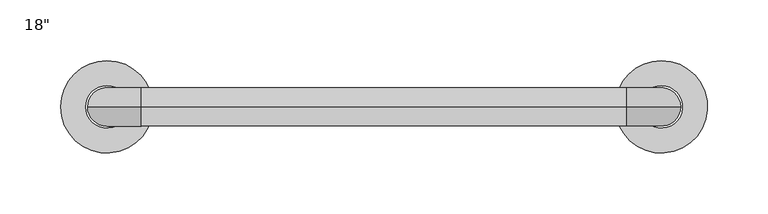
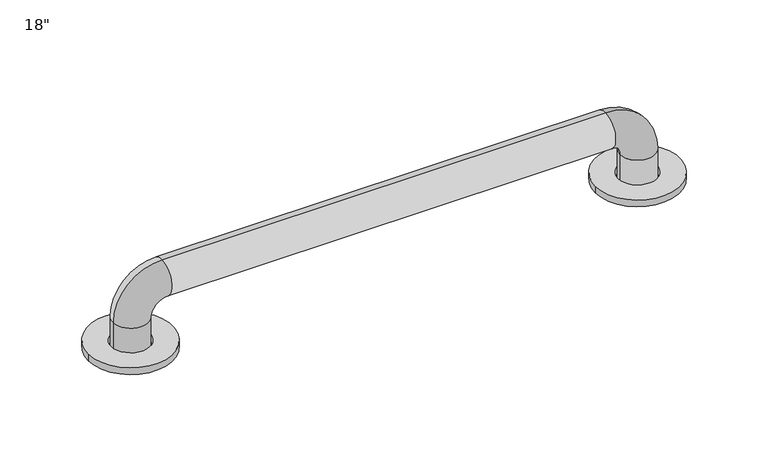
"""IFC4 building model written with IfcOpenShell, lengths in millimetres: proxy geometry."""

from ifc_helpers import new_model, si_unit, point, frame, frame_2d, origin, origin_with_axes, origin_2d, place, context, project, spatial, circle_curve, ellipse_curve, trimmed, segment, composite_curve, outline, extrude, source, transform, mapped, element, save
from ifc_brep_helpers import plane_surface, cylinder_surface, revolved_surface, advanced_brep


def proxy_37aad3db(model_context):
    return source(origin(), model_context, "Body", "SolidModel", [
        extrude(outline(composite_curve([segment(trimmed(circle_curve(frame_2d((457.2, 0.0)), 38.1), [point((419.1, 0.0))], [point((457.2, 38.1))], False, "CARTESIAN"), True, "CONTINUOUS"), segment(trimmed(circle_curve(frame_2d((457.2, 0.0)), 38.1), [point((457.2, 38.1))], [point((419.1, 0.0))], False, "CARTESIAN"), True, "CONTINUOUS")], self_intersect=False), holes=[composite_curve([segment(trimmed(circle_curve(frame_2d((457.2, 0.0)), 17.4625), [point((439.7375, 0.0))], [point((457.2, 17.4625))], True, "CARTESIAN"), True, "CONTINUOUS"), segment(trimmed(circle_curve(frame_2d((457.2, 0.0)), 17.4625), [point((457.2, 17.4625))], [point((439.7375, 0.0))], True, "CARTESIAN"), True, "CONTINUOUS")], self_intersect=False)]), origin_with_axes(), (0.0, 0.0, 1.0), 6.35),
        extrude(outline(composite_curve([segment(trimmed(circle_curve(origin_2d(), 38.1), [point((-38.1, 0.0))], [point((0.0, 38.1))], False, "CARTESIAN"), True, "CONTINUOUS"), segment(trimmed(circle_curve(origin_2d(), 38.1), [point((0.0, 38.1))], [point((-38.1, 0.0))], False, "CARTESIAN"), True, "CONTINUOUS")], self_intersect=False), holes=[composite_curve([segment(trimmed(circle_curve(origin_2d(), 17.4625), [point((-17.4625, 0.0))], [point((0.0, 17.4625))], True, "CARTESIAN"), True, "CONTINUOUS"), segment(trimmed(circle_curve(origin_2d(), 17.4625), [point((0.0, 17.4625))], [point((-17.4625, 0.0))], True, "CARTESIAN"), True, "CONTINUOUS")], self_intersect=False)]), origin_with_axes(), (0.0, 0.0, 1.0), 6.35),
        advanced_brep(
        [(473.075, 0.0, 0.0), (441.325, 0.0, 0.0), (441.325, 0.0, 28.575), (473.075, 0.0, 28.575), (428.625, 0.0, 41.275), (428.625, 0.0, 73.025), (28.575, 0.0, 41.275), (28.575, 0.0, 73.025), (15.875, 0.0, 28.575), (-15.875, 0.0, 28.575), (-15.875, 0.0, 0.0), (15.875, 0.0, 0.0)],
        [
            (0, 1, circle_curve(frame((457.2, 0.0, 0.0), z_axis=(0.0, 0.0, -1.0), x_axis=(-1.0, 0.0, 0.0)), 15.875)),
            (1, 0, circle_curve(frame((457.2, 0.0, 0.0), z_axis=(0.0, 0.0, -1.0), x_axis=(-1.0, 0.0, 0.0)), 15.875)),
            (1, 2),
            (2, 3, circle_curve(frame((457.2, 0.0, 28.575), z_axis=(0.0, 0.0, -1.0), x_axis=(-1.0, 0.0, 0.0)), 15.875)),
            (3, 0),
            (3, 2, circle_curve(frame((457.2, 0.0, 28.575), z_axis=(0.0, 0.0, -1.0), x_axis=(-1.0, 0.0, 0.0)), 15.875)),
            (4, 5, circle_curve(frame((428.625, 0.0, 57.15), z_axis=(1.0, 0.0, 0.0), x_axis=(0.0, 0.0, -1.0)), 15.875)),
            (5, 3, circle_curve(frame((428.625, 0.0, 28.575), z_axis=(0.0, 1.0, 0.0), x_axis=(1.0, 0.0, 0.0)), 44.45)),
            (2, 4, circle_curve(frame((428.625, 0.0, 28.575), z_axis=(0.0, -1.0, 0.0), x_axis=(1.0, 0.0, 0.0)), 12.7)),
            (5, 4, circle_curve(frame((428.625, 0.0, 57.15), z_axis=(1.0, 0.0, 0.0), x_axis=(0.0, 0.0, -1.0)), 15.875)),
            (4, 6),
            (6, 7, circle_curve(frame((28.575, 0.0, 57.15), z_axis=(1.0, 0.0, 0.0), x_axis=(0.0, 0.0, -1.0)), 15.875)),
            (7, 5),
            (7, 6, circle_curve(frame((28.575, 0.0, 57.15), z_axis=(1.0, 0.0, 0.0), x_axis=(0.0, 0.0, -1.0)), 15.875)),
            (8, 9, circle_curve(frame((0.0, 0.0, 28.575), z_axis=(0.0, 0.0, 1.0), x_axis=(1.0, 0.0, 0.0)), 15.875)),
            (9, 7, circle_curve(frame((28.575, 0.0, 28.575), z_axis=(0.0, 1.0, 0.0), x_axis=(0.0, 0.0, 1.0)), 44.45)),
            (6, 8, circle_curve(frame((28.575, 0.0, 28.575), z_axis=(0.0, -1.0, 0.0), x_axis=(0.0, 0.0, 1.0)), 12.7)),
            (9, 8, circle_curve(frame((0.0, 0.0, 28.575), z_axis=(0.0, 0.0, 1.0), x_axis=(1.0, 0.0, 0.0)), 15.875)),
            (10, 11, circle_curve(frame((0.0, 0.0, 0.0), z_axis=(0.0, 0.0, -1.0), x_axis=(1.0, 0.0, 0.0)), 15.875)),
            (11, 10, circle_curve(frame((0.0, 0.0, 0.0), z_axis=(0.0, 0.0, -1.0), x_axis=(1.0, 0.0, 0.0)), 15.875)),
            (8, 11),
            (10, 9),
        ],
        [
            plane_surface(frame((457.2, 0.0, 0.0), z_axis=(0.0, 0.0, -1.0), x_axis=(0.0, 1.0, 0.0))),
            cylinder_surface(frame((457.2, 0.0, 0.0), z_axis=(0.0, 0.0, -1.0), x_axis=(-1.0, 0.0, 0.0)), 15.875),
            revolved_surface(trimmed(ellipse_curve(frame((457.2, 0.0, 28.575), z_axis=(0.0, 0.0, 1.0), x_axis=(-1.0, 0.0, 0.0)), 15.875, 15.875), [point((473.075, 0.0, 28.575))], [point((441.325, 0.0, 28.575))], True, "CARTESIAN"), (428.625, 0.0, 28.575), (0.0, 1.0, 0.0)),
            revolved_surface(trimmed(ellipse_curve(frame((457.2, 0.0, 28.575), z_axis=(0.0, 0.0, 1.0), x_axis=(-1.0, 0.0, 0.0)), 15.875, 15.875), [point((441.325, 0.0, 28.575))], [point((473.075, 0.0, 28.575))], True, "CARTESIAN"), (428.625, 0.0, 28.575), (0.0, 1.0, 0.0)),
            cylinder_surface(frame((428.625, 0.0, 57.15), z_axis=(1.0, 0.0, 0.0), x_axis=(0.0, 0.0, -1.0)), 15.875),
            revolved_surface(trimmed(ellipse_curve(frame((28.575, 0.0, 57.15), z_axis=(-1.0, 0.0, 0.0), x_axis=(0.0, 0.0, -1.0)), 15.875, 15.875), [point((28.575, 0.0, 73.025))], [point((28.575, 0.0, 41.275))], True, "CARTESIAN"), (28.575, 0.0, 28.575), (0.0, 1.0, 0.0)),
            revolved_surface(trimmed(ellipse_curve(frame((28.575, 0.0, 57.15), z_axis=(-1.0, 0.0, 0.0), x_axis=(0.0, 0.0, -1.0)), 15.875, 15.875), [point((28.575, 0.0, 41.275))], [point((28.575, 0.0, 73.025))], True, "CARTESIAN"), (28.575, 0.0, 28.575), (0.0, 1.0, 0.0)),
            plane_surface(frame((0.0, 0.0, 0.0), z_axis=(0.0, 0.0, -1.0), x_axis=(0.0, 1.0, 0.0))),
            cylinder_surface(frame((0.0, 0.0, 28.575), z_axis=(0.0, 0.0, 1.0), x_axis=(1.0, 0.0, 0.0)), 15.875),
        ],
        [
            (0, [[1, 2]]),
            (1, [[3, 4, 5, -2]]),
            (1, [[-5, 6, -3, -1]]),
            (2, [[7, 8, -4, 9]]),
            (3, [[10, -9, -6, -8]]),
            (4, [[11, 12, 13, -7]]),
            (4, [[-13, 14, -11, -10]]),
            (5, [[15, 16, -12, 17]]),
            (6, [[18, -17, -14, -16]]),
            (7, [[19, 20]]),
            (8, [[21, -19, 22, -15]]),
            (8, [[-22, -20, -21, -18]]),
        ],
    ),
    ])


if __name__ == "__main__":
    model = new_model("IFC4")
    model_context = context("Model", 3, world=origin())
    ifc_project = project(units=[si_unit("LENGTHUNIT", "METRE", prefix="MILLI")], contexts=[model_context])
    site = spatial("IfcSite", under=ifc_project)
    building = spatial("IfcBuilding", under=site)
    placement = place(None, origin())
    proxy_shape = proxy_37aad3db(model_context)
    element("IfcBuildingElementProxy", 1, Name="Seqm-Grab Bar : 18\"", ObjectType="Seqm-Grab Bar : 18\"", at=placement, inside=building, context=model_context, shape_type="MappedRepresentation", body=[
        mapped(proxy_shape, transform((0.0, 0.0, 0.0), x_axis=(1.0, 0.0, 0.0), y_axis=(0.0, 1.0, 0.0), z_axis=(0.0, 0.0, 1.0))),
    ])
    save(model, "model.ifc")

# Revit data of these elements
# Type "Seqm-Grab Bar : 18\""
#   Spec Number = "10 28 00"
#   Spec Description = "18\" GRAB BAR"
#   Length = 1' - 6"
#   Default Elevation = 4' - 0"
#   Grab Bar Material = GRAB BARS - AT ADA RESTROOMS ONLY
# Element 1 (IfcBuildingElementProxy, "Seqm-Grab Bar : 18\"")
#   Materials on its faces: "GRAB BARS - AT ADA RESTROOMS ONLY"
# Materials
#   "GRAB BARS - AT ADA RESTROOMS ONLY": class "Generic", colour RGB 120 120 120, transparency 0, Cost = 0
